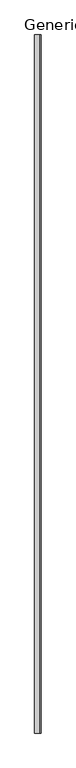
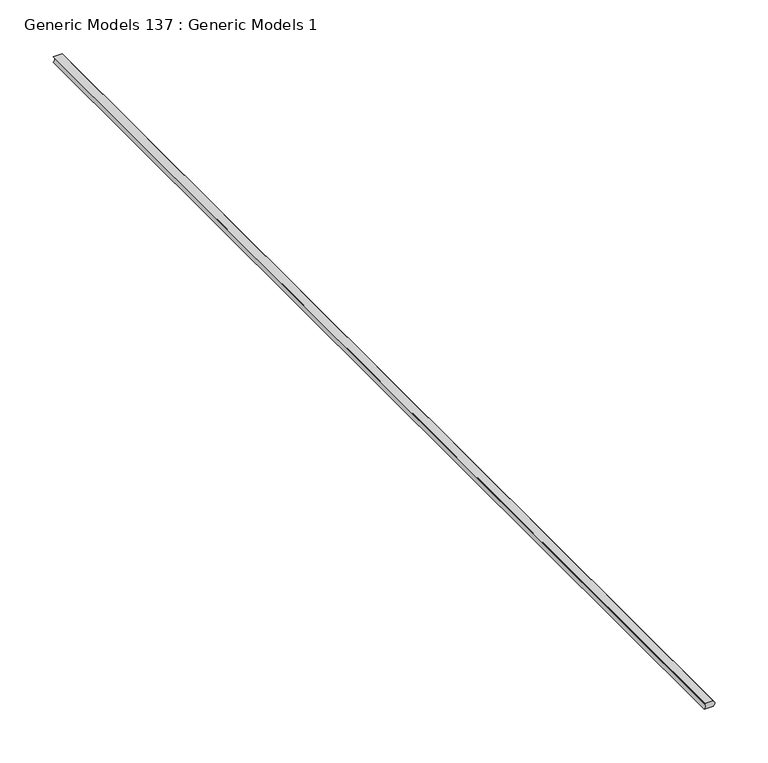
"""IFC4 building model written with IfcOpenShell, lengths in millimetres: proxy geometry, Generic Models 137 : Generic Models 1."""

from ifc_helpers import new_model, si_unit, point, frame, frame_2d, origin, place, context, project, spatial, polyline, circle_curve, trimmed, segment, composite_curve, outline, extrude, source, transform, mapped, element, save


def generic_models_137_generic_models_1_a64e1080(model_context):
    return source(origin(), model_context, "Body", "SweptSolid", [
        extrude(outline(composite_curve([segment(polyline([(-2150.4233876, 50916.7994166), (-2150.4233876, 50926.3244166)]), True, "CONTINUOUS"), segment(trimmed(circle_curve(frame_2d((-2147.2483876, 50923.4096762)), 4.3100275), [point((-2150.4233876, 50926.3244166))], [point((-2144.0733876, 50926.3244166))], False, "CARTESIAN"), True, "CONTINUOUS"), segment(polyline([(-2144.0733876, 50926.3244166), (-2144.0733876, 50916.7994166)]), True, "CONTINUOUS"), segment(trimmed(circle_curve(frame_2d((-2147.2483876, 50913.8846762)), 4.3100275), [point((-2144.0733876, 50916.7994166))], [point((-2150.4233876, 50916.7994166))], True, "CARTESIAN"), True, "CONTINUOUS")], self_intersect=False)), frame((0.0, 0.0, 0.0), z_axis=(0.0, 1.0, 0.0), x_axis=(0.0, 0.0, 1.0)), (0.0, 0.0, 1.0), 1219.2),
    ])


if __name__ == "__main__":
    model = new_model("IFC4")
    model_context = context("Model", 3, world=origin())
    ifc_project = project(units=[si_unit("LENGTHUNIT", "METRE", prefix="MILLI")], contexts=[model_context])
    site = spatial("IfcSite", under=ifc_project)
    building = spatial("IfcBuilding", under=site)
    placement = place(None, origin())
    generic_models_137_generic_models_1_shape = generic_models_137_generic_models_1_a64e1080(model_context)
    element("IfcBuildingElementProxy", 1, Name="Generic Models 137 : Generic Models 1", ObjectType="Generic Models 137 : Generic Models 1", at=placement, inside=building, context=model_context, shape_type="MappedRepresentation", body=[
        mapped(generic_models_137_generic_models_1_shape, transform((0.0, 0.0, 0.0), x_axis=(1.0, 0.0, 0.0), y_axis=(0.0, 1.0, 0.0), z_axis=(0.0, 0.0, 1.0))),
    ])
    save(model, "model.ifc")

# Revit data of these elements
# Element 1 (IfcBuildingElementProxy, "Generic Models 137 : Generic Models 1")
#   Materials on its faces: "SEALANT (W/ BACKER ROD IF NECESSARY)"
# Materials
#   "SEALANT (W/ BACKER ROD IF NECESSARY)": class "Unassigned", colour RGB 120 120 120, transparency 0, Cost = 0
